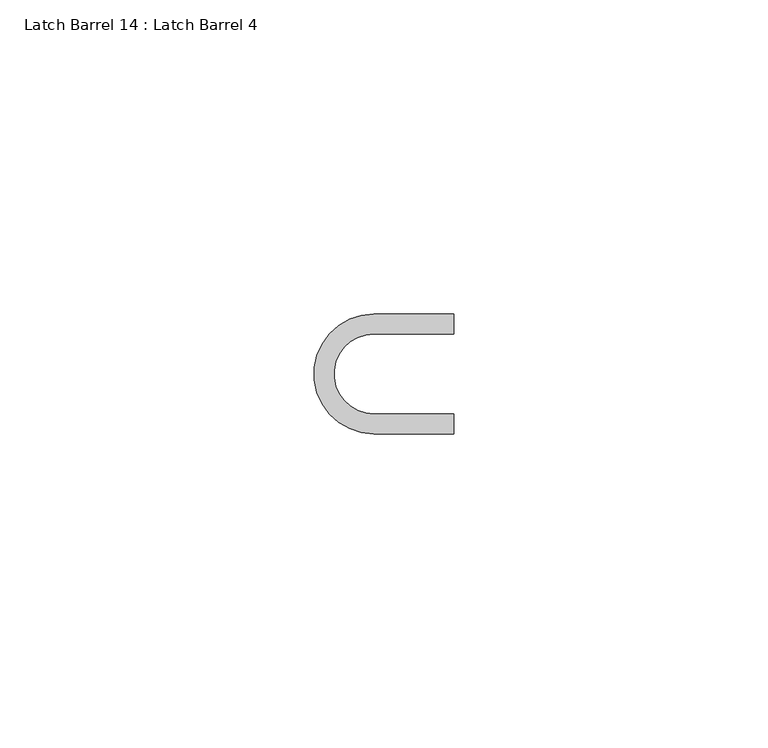
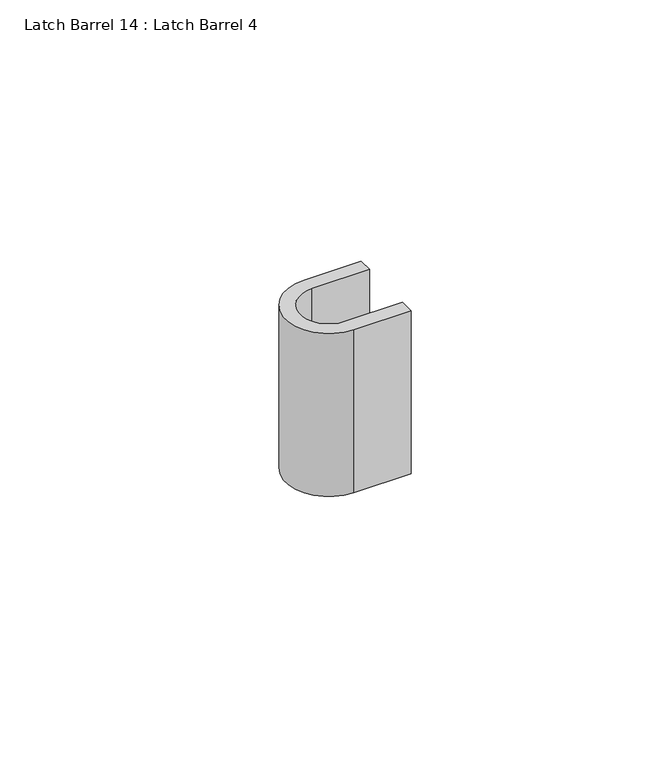
"""IFC4 building model written with IfcOpenShell, lengths in millimetres: proxy geometry, Latch Barrel 14 : Latch Barrel 4."""

from ifc_helpers import new_model, si_unit, point, frame, frame_2d, origin, place, context, project, spatial, polyline, circle_curve, trimmed, segment, composite_curve, outline, extrude, source, transform, mapped, element, save


def latch_barrel_14_latch_barrel_4_f3fd6b15(model_context):
    return source(origin(), model_context, "Body", "SweptSolid", [
        extrude(outline(composite_curve([segment(trimmed(circle_curve(frame_2d((587309.5435739, -532839.3663841)), 6.35), [point((587309.5435739, -532833.0163841))], [point((587309.5435739, -532845.7163841))], True, "CARTESIAN"), True, "CONTINUOUS"), segment(polyline([(587309.5435739, -532845.7163841), (587322.2435739, -532845.7163841), (587322.2435739, -532848.8913841), (587309.5435739, -532848.8913841)]), True, "CONTINUOUS"), segment(trimmed(circle_curve(frame_2d((587309.5435739, -532839.3663841)), 9.525), [point((587309.5435739, -532848.8913841))], [point((587309.5435739, -532829.8413841))], False, "CARTESIAN"), True, "CONTINUOUS"), segment(polyline([(587309.5435739, -532829.8413841), (587322.2435739, -532829.8413841), (587322.2435739, -532833.0163841), (587309.5435739, -532833.0163841)]), True, "CONTINUOUS")], self_intersect=False)), frame((0.0, 0.0, 50.8), z_axis=(0.0, 0.0, 1.0), x_axis=(1.0, 0.0, 0.0)), (0.0, 0.0, 1.0), 38.1),
    ])


if __name__ == "__main__":
    model = new_model("IFC4")
    model_context = context("Model", 3, world=origin())
    ifc_project = project(units=[si_unit("LENGTHUNIT", "METRE", prefix="MILLI")], contexts=[model_context])
    site = spatial("IfcSite", under=ifc_project)
    building = spatial("IfcBuilding", under=site)
    placement = place(None, origin())
    latch_barrel_14_latch_barrel_4_shape = latch_barrel_14_latch_barrel_4_f3fd6b15(model_context)
    element("IfcBuildingElementProxy", 1, Name="Latch Barrel 14 : Latch Barrel 4", ObjectType="Latch Barrel 14 : Latch Barrel 4", at=placement, inside=building, context=model_context, shape_type="MappedRepresentation", body=[
        mapped(latch_barrel_14_latch_barrel_4_shape, transform((0.0, 0.0, 0.0), x_axis=(1.0, 0.0, 0.0), y_axis=(0.0, 1.0, 0.0), z_axis=(0.0, 0.0, 1.0))),
    ])
    save(model, "model.ifc")

# Revit data of these elements
# Element 1 (IfcBuildingElementProxy, "Latch Barrel 14 : Latch Barrel 4")
#   Materials on its faces: "GALV. SLIDE BOLT"
# Materials
#   "GALV. SLIDE BOLT": class "Metal", colour RGB 189 187 185, transparency 0, Description = "Carbon steel", Cost = 0
